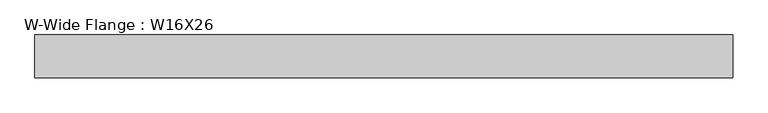
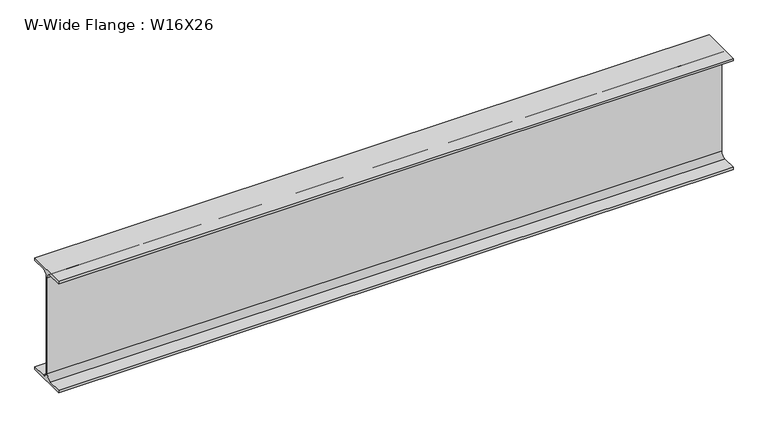
"""IFC4 building model written with IfcOpenShell, lengths in millimetres: beam geometry, W-Wide Flange : W16X26."""

from ifc_helpers import new_model, si_unit, point, frame, frame_2d, origin, place, context, project, spatial, polyline, circle_curve, trimmed, segment, composite_curve, outline, extrude, source, transform, mapped, element, save


def w_wide_flange_w16x26_d8ea63e7(model_context):
    return source(origin(), model_context, "Body", "SweptSolid", [
        extrude(outline(composite_curve([segment(polyline([(-69.85, -190.5496094), (-21.43125, -190.5496094)]), True, "CONTINUOUS"), segment(trimmed(circle_curve(frame_2d((-21.43125, -172.2933594)), 18.25625), [point((-21.43125, -190.5496094))], [point((-3.175, -172.2933594))], True, "CARTESIAN"), True, "CONTINUOUS"), segment(polyline([(-3.175, -172.2933594), (-3.175, 172.2933594)]), True, "CONTINUOUS"), segment(trimmed(circle_curve(frame_2d((-21.43125, 172.2933594)), 18.25625), [point((-3.175, 172.2933594))], [point((-21.43125, 190.5496094))], True, "CARTESIAN"), True, "CONTINUOUS"), segment(polyline([(-21.43125, 190.5496094), (-69.85, 190.5496094), (-69.85, 199.2808594), (69.85, 199.2808594), (69.85, 190.5496094), (21.43125, 190.5496094)]), True, "CONTINUOUS"), segment(trimmed(circle_curve(frame_2d((21.43125, 172.2933594)), 18.25625), [point((21.43125, 190.5496094))], [point((3.175, 172.2933594))], True, "CARTESIAN"), True, "CONTINUOUS"), segment(polyline([(3.175, 172.2933594), (3.175, -172.2933594)]), True, "CONTINUOUS"), segment(trimmed(circle_curve(frame_2d((21.43125, -172.2933594)), 18.25625), [point((3.175, -172.2933594))], [point((21.43125, -190.5496094))], True, "CARTESIAN"), True, "CONTINUOUS"), segment(polyline([(21.43125, -190.5496094), (69.85, -190.5496094), (69.85, -199.2808594), (-69.85, -199.2808594), (-69.85, -190.5496094)]), True, "CONTINUOUS")], self_intersect=False)), frame((-1079.5, 0.0, 0.0), z_axis=(1.0, 0.0, 0.0), x_axis=(0.0, 1.0, 0.0)), (0.0, 0.0, 1.0), 2284.7779979),
    ])


if __name__ == "__main__":
    model = new_model("IFC4")
    model_context = context("Model", 3, world=origin())
    ifc_project = project(units=[si_unit("LENGTHUNIT", "METRE", prefix="MILLI")], contexts=[model_context])
    site = spatial("IfcSite", under=ifc_project)
    building = spatial("IfcBuilding", under=site)
    placement = place(None, origin())
    w_wide_flange_w16x26_shape = w_wide_flange_w16x26_d8ea63e7(model_context)
    element("IfcBeam", 1, ObjectType="W-Wide Flange : W16X26", at=placement, inside=building, context=model_context, shape_type="MappedRepresentation", body=[
        mapped(w_wide_flange_w16x26_shape, transform((0.0, 0.0, 0.0), x_axis=(1.0, 0.0, 0.0), y_axis=(0.0, 1.0, 0.0), z_axis=(0.0, 0.0, 1.0))),
    ])
    save(model, "model.ifc")

# Revit data of these elements
# Type "W-Wide Flange : W16X26"
#   Assembly Code = "B10"
#   W = 26
#   Start Extension Calculation [instance default] = 10' - 0"
#   Start Extension [instance default] = -0' - 0 1/2"
#   End Extension Calculation [instance default] = 10' - 0"
#   End Extension [instance default] = -0' - 0 1/2"
#   Length [instance default] = 5' - 0"
#   bf = 0' - 5 1/2"
#   d = 1' - 3 177/256"
#   k = 0' - 1 1/16"
#   k2 = 0' - 0 23/32"
#   tf = 0' - 0 11/32"
#   tw = 0' - 0 1/4"
#   A = 0.05 SF
#   Beam Material [instance default] = Metal - Steel - ASTM A992
# Element 1 (IfcBeam, "W-Wide Flange : W16X26")
#   End Extension Calculation = 9' - 11.45189"
#   End Extension = -0' - 1.04811"
#   Materials on its faces: "Metal - Steel - ASTM A992"
# Materials
#   "Metal - Steel - ASTM A992": class "Metal", colour RGB 128 0 0, transparency 0
